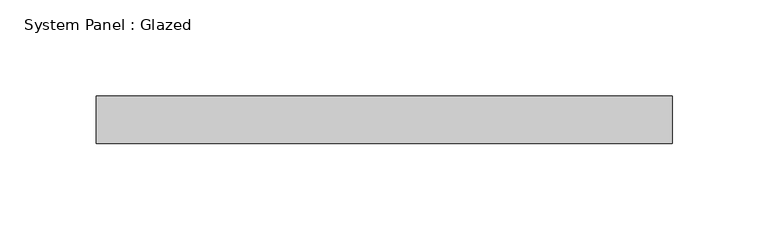
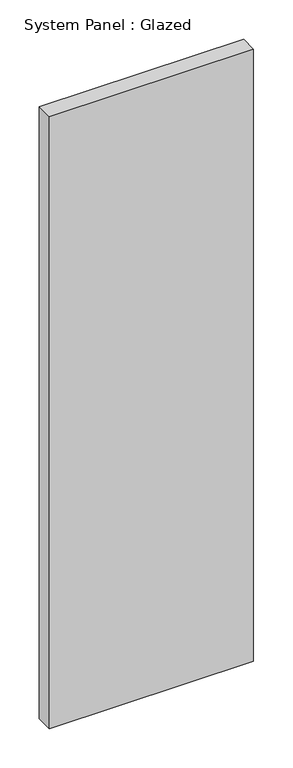
"""IFC4 building model written with IfcOpenShell, lengths in millimetres: plate geometry, System Panel : Glazed."""

from ifc_helpers import new_model, si_unit, origin, origin_with_axes, place, context, project, spatial, polyline, outline, extrude, source, transform, mapped, element, save


def system_panel_glazed_abe8033e(model_context):
    return source(origin(), model_context, "Body", "SweptSolid", [
        extrude(outline(polyline([(150.0, 24.5), (-150.0, 24.5), (-150.0, 49.5), (150.0, 49.5), (150.0, 24.5)])), origin_with_axes(), (0.0, 0.0, 1.0), 950.0),
    ])


if __name__ == "__main__":
    model = new_model("IFC4")
    model_context = context("Model", 3, world=origin())
    ifc_project = project(units=[si_unit("LENGTHUNIT", "METRE", prefix="MILLI")], contexts=[model_context])
    site = spatial("IfcSite", under=ifc_project)
    building = spatial("IfcBuilding", under=site)
    placement = place(None, origin())
    system_panel_glazed_shape = system_panel_glazed_abe8033e(model_context)
    element("IfcPlate", 1, ObjectType="System Panel : Glazed", at=placement, inside=building, context=model_context, shape_type="MappedRepresentation", body=[
        mapped(system_panel_glazed_shape, transform((0.0, 0.0, 0.0), x_axis=(1.0, 0.0, 0.0), y_axis=(0.0, 1.0, 0.0), z_axis=(0.0, 0.0, 1.0))),
    ])
    save(model, "model.ifc")

# Revit data of these elements
# Element 1 (IfcPlate, "System Panel : Glazed")
#   Materials on its faces: "Glass"
# Materials
#   "Glass": class "Glass", colour RGB 218 227 224, transparency 0.85, Description = "Soda Lime Glass", Cost = 0
